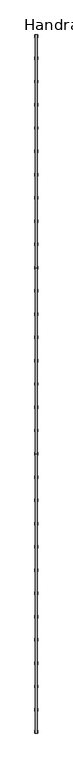
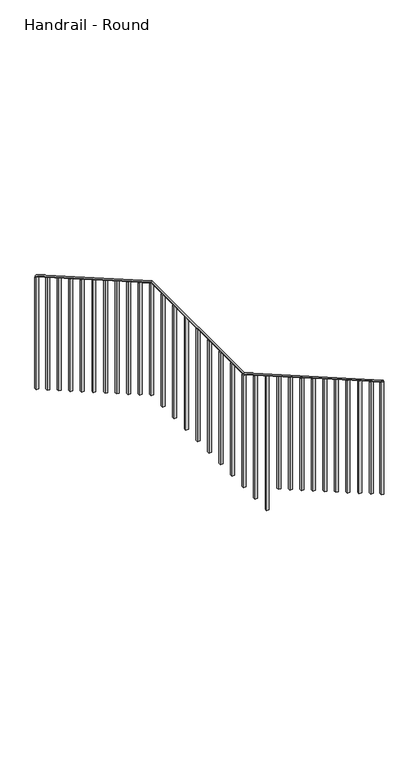
"""IFC4 building model written with IfcOpenShell, lengths in millimetres: railing geometry, Handrail - Round."""

import ifcopenshell
import ifcopenshell.guid

model = None  # the IFC model being written
_history = None  # IfcOwnerHistory: only IFC2X3 demands one
_inside = {}  # id of a spatial element -> (the spatial element, [elements in it])
_under = {}  # id of a project, library or spatial element -> (it, [spatial elements below it])
_declared = {}  # id of a project -> (the project, [libraries it declares])
_typed = {}  # id of a type object -> (the type object, [elements of that type])
_made_of = {}  # id of a material, layer set ... -> (it, [elements and type objects made of it])


def new_model(schema):
    """Start an empty IFC model of exactly this schema.

    Asked for "IFC4X3", IfcOpenShell would pick the latest addendum, in which some entities
    have other attributes; the version numbers below select the first issue.
    IFC2X3 requires an IfcOwnerHistory on every rooted entity: one is made here for all.
    """
    global model, _history
    if schema == "IFC4X3":
        model = ifcopenshell.file(schema_version=(4, 3, 0, 0))
    else:
        model = ifcopenshell.file(schema=schema)
    _inside.clear()
    _under.clear()
    _declared.clear()
    _typed.clear()
    _made_of.clear()
    _history = None
    if model.schema == "IFC2X3":
        org = make("IfcOrganization", Name="unknown")
        user = make(
            "IfcPersonAndOrganization",
            ThePerson=make("IfcPerson", FamilyName="unknown"),
            TheOrganization=org,
        )
        app = make(
            "IfcApplication",
            ApplicationDeveloper=org,
            Version="unknown",
            ApplicationFullName="unknown",
            ApplicationIdentifier="unknown",
        )
        _history = make(
            "IfcOwnerHistory",
            OwningUser=user,
            OwningApplication=app,
            ChangeAction="ADDED",
            CreationDate=0,
        )
    return model


def make(cls, **values):
    """One entity of the class cls with the attributes given. An attribute that is None is left unset."""
    return model.create_entity(
        cls, **{name: value for name, value in values.items() if value is not None}
    )


def rooted(cls, **values):
    """An entity with a GlobalId (a new one), such as an element, a storey or a relation."""
    return make(cls, GlobalId=ifcopenshell.guid.new(), OwnerHistory=_history, **values)


def si_unit(unit_type, name, prefix=None):
    """IfcSIUnit, for example si_unit("LENGTHUNIT", "METRE", prefix="MILLI")."""
    return make("IfcSIUnit", UnitType=unit_type, Prefix=prefix, Name=name)


def assignment(units):
    """IfcUnitAssignment: the units of a project."""
    return None if units is None else make("IfcUnitAssignment", Units=units)


def point(xyz):
    """IfcCartesianPoint."""
    return None if xyz is None else make("IfcCartesianPoint", Coordinates=xyz)


def direction(xyz):
    """IfcDirection."""
    return None if xyz is None else make("IfcDirection", DirectionRatios=xyz)


def frame(location, z_axis=None, x_axis=None):
    """IfcAxis2Placement3D, a coordinate frame: its origin and axes. An axis left out is left unset."""
    return make(
        "IfcAxis2Placement3D",
        Location=point(location),
        Axis=direction(z_axis),
        RefDirection=direction(x_axis),
    )


def origin():
    """The frame at (0, 0, 0) with its axes left unset."""
    return frame((0.0, 0.0, 0.0))


def place(relative_to, where):
    """IfcLocalPlacement: puts the frame where relative to a parent placement (None: the world)."""
    return make(
        "IfcLocalPlacement", PlacementRelTo=relative_to, RelativePlacement=where
    )


def context(
    kind, dimensions, precision=None, world=None, true_north=None, identifier=None
):
    """IfcGeometricRepresentationContext, for example the 3D "Model" context."""
    return make(
        "IfcGeometricRepresentationContext",
        ContextIdentifier=identifier,
        ContextType=kind,
        CoordinateSpaceDimension=dimensions,
        Precision=precision,
        WorldCoordinateSystem=world,
        TrueNorth=true_north,
    )


def project(units=None, contexts=None):
    """IfcProject with its units and contexts."""
    return rooted(
        "IfcProject",
        Name="project",
        RepresentationContexts=contexts,
        UnitsInContext=assignment(units),
    )


def spatial(cls, under=None, at=None, **own):
    """A site, building, storey or space (cls), placed at a placement, below another one or the project."""
    s = rooted(cls, ObjectPlacement=at, **own)
    if under is not None:
        _under.setdefault(under.id(), (under, []))[1].append(s)
    return s


def polyline(points):
    """IfcPolyline through the points."""
    return make("IfcPolyline", Points=[point(p) for p in points])


def ellipse_curve(where, semi_axis1, semi_axis2):
    """IfcEllipse in the frame where."""
    return make(
        "IfcEllipse", Position=where, SemiAxis1=semi_axis1, SemiAxis2=semi_axis2
    )


def outline(outer, holes=None, kind="AREA"):
    """IfcArbitraryClosedProfileDef: a profile drawn as a closed curve; with holes, ...WithVoids."""
    if holes is None:
        return make("IfcArbitraryClosedProfileDef", ProfileType=kind, OuterCurve=outer)
    return make(
        "IfcArbitraryProfileDefWithVoids",
        ProfileType=kind,
        OuterCurve=outer,
        InnerCurves=holes,
    )


def extrude(swept, where, along, depth):
    """IfcExtrudedAreaSolid: the profile swept, set in the frame where, extruded along a direction by depth."""
    return make(
        "IfcExtrudedAreaSolid",
        SweptArea=swept,
        Position=where,
        ExtrudedDirection=direction(along),
        Depth=depth,
    )


def shape(context_of_items, identifier, shape_type, items):
    """IfcShapeRepresentation: the items that make up one representation, for example the "Body"."""
    return make(
        "IfcShapeRepresentation",
        ContextOfItems=context_of_items,
        RepresentationIdentifier=identifier,
        RepresentationType=shape_type,
        Items=items,
    )


def source(mapping_origin, context_of_items, identifier, shape_type, items):
    """IfcRepresentationMap: a shape defined once, which mapped items show again and again."""
    return make(
        "IfcRepresentationMap",
        MappingOrigin=mapping_origin,
        MappedRepresentation=shape(context_of_items, identifier, shape_type, items),
    )


def transform(
    local_origin,
    x_axis=None,
    y_axis=None,
    z_axis=None,
    scale=None,
    scale2=None,
    scale3=None,
    uniform=True,
):
    """IfcCartesianTransformationOperator3D, or its non-uniform kind. x_axis, y_axis, z_axis: its Axis1, 2, 3."""
    if uniform:
        return make(
            "IfcCartesianTransformationOperator3D",
            Axis1=direction(x_axis),
            Axis2=direction(y_axis),
            LocalOrigin=point(local_origin),
            Scale=scale,
            Axis3=direction(z_axis),
        )
    return make(
        "IfcCartesianTransformationOperator3DnonUniform",
        Axis1=direction(x_axis),
        Axis2=direction(y_axis),
        LocalOrigin=point(local_origin),
        Scale=scale,
        Axis3=direction(z_axis),
        Scale2=scale2,
        Scale3=scale3,
    )


def mapped(mapping_source, mapping_target):
    """IfcMappedItem: shows the shape of a source again, moved by a transform."""
    return make(
        "IfcMappedItem", MappingSource=mapping_source, MappingTarget=mapping_target
    )


def made_of(thing, what):
    """Note that an element or type object is made of a material, layer set ...; save() writes the relation."""
    if what is not None:
        _made_of.setdefault(what.id(), (what, []))[1].append(thing)
    return thing


def element(
    cls,
    number,
    at=None,
    inside=None,
    cuts=None,
    type_object=None,
    material=None,
    context=None,
    identifier="Body",
    shape_type=None,
    held_by="IfcProductDefinitionShape",
    body=None,
    shapes=None,
    **own,
):
    """One element of the class cls, such as IfcWall. Its Tag is "e" and its number.

    at: its placement. inside: the storey or other place that contains it. cuts: it is an
    opening in that element (IfcRelVoidsElement). A single representation is given by context,
    identifier, shape_type and body (its items); several are given by shapes. held_by: the class
    of the entity that holds the representations. save() writes the other relations.
    """
    e = rooted(cls, Tag="e%d" % number, ObjectPlacement=at, **own)
    if body is not None:
        shapes = [shape(context, identifier, shape_type, body)]
    if shapes is not None:
        e.Representation = make(held_by, Representations=shapes)
    if inside is not None:
        _inside.setdefault(inside.id(), (inside, []))[1].append(e)
    if cuts is not None:
        rooted(
            "IfcRelVoidsElement", RelatingBuildingElement=cuts, RelatedOpeningElement=e
        )
    if type_object is not None:
        _typed.setdefault(type_object.id(), (type_object, []))[1].append(e)
    return made_of(e, material)


def aggregate(whole, parts):
    """IfcRelAggregates: a whole, such as a stair, and the parts it consists of."""
    return rooted("IfcRelAggregates", RelatingObject=whole, RelatedObjects=parts)


def save(model, path):
    """Write the relations noted so far, then the file.

    IfcRelAggregates (storeys below a building ...), IfcRelContainedInSpatialStructure (elements
    in a storey), IfcRelDefinesByType, IfcRelAssociatesMaterial and IfcRelDeclares: one each for
    every whole, place, type object, material and project.
    """
    for whole, parts in _under.values():
        aggregate(whole, parts)
    for where, things in _inside.values():
        rooted(
            "IfcRelContainedInSpatialStructure",
            RelatedElements=things,
            RelatingStructure=where,
        )
    for kind, things in _typed.values():
        rooted("IfcRelDefinesByType", RelatedObjects=things, RelatingType=kind)
    for what, things in _made_of.values():
        rooted("IfcRelAssociatesMaterial", RelatedObjects=things, RelatingMaterial=what)
    for by, libraries in _declared.values():
        rooted("IfcRelDeclares", RelatingContext=by, RelatedDefinitions=libraries)
    model.write(path)


def plane_surface(at):
    """IfcPlane: the flat surface through the origin of the frame at, square to its z axis."""
    return make("IfcPlane", Position=at)


def cylinder_surface(at, radius):
    """IfcCylindricalSurface: all points at the distance radius from the z axis of the frame at."""
    return make("IfcCylindricalSurface", Position=at, Radius=radius)


def advanced_brep(points, edges, surfaces, faces):
    """IfcAdvancedBrep: a solid bounded by faces that lie on surfaces and meet in shared edges.

    An edge is (start, end): straight between two places in points (the first is 0);
    or (start, end, curve); or (start, end, curve, False) where it runs against its curve.
    A face is (place in surfaces, loops), or (place, loops, False) where it looks against
    its surface's normal. A loop lists edges by number (the first is 1), with a minus sign
    where the edge is run from its end to its start. The first loop is the outer one.
    """
    corners = [point(p) for p in points]
    vertices = [make("IfcVertexPoint", VertexGeometry=c) for c in corners]
    made = []
    for start, end, *more in edges:
        made.append(
            make(
                "IfcEdgeCurve",
                EdgeStart=vertices[start],
                EdgeEnd=vertices[end],
                EdgeGeometry=more[0] if more else make("IfcPolyline", Points=[corners[start], corners[end]]),
                SameSense=more[1] if len(more) > 1 else True,
            )
        )
    hull = []
    for where, loops, *sense in faces:
        bounds = []
        for j, loop in enumerate(loops):
            ring = [make("IfcOrientedEdge", EdgeElement=made[abs(k) - 1], Orientation=k > 0) for k in loop]
            bounds.append(
                make(
                    "IfcFaceOuterBound" if j == 0 else "IfcFaceBound",
                    Bound=make("IfcEdgeLoop", EdgeList=ring),
                    Orientation=True,
                )
            )
        hull.append(make("IfcAdvancedFace", Bounds=bounds, FaceSurface=surfaces[where], SameSense=sense[0] if sense else True))
    return make("IfcAdvancedBrep", Outer=make("IfcClosedShell", CfsFaces=hull))


def handrail_round_a1da8104(model_context):
    return source(origin(), model_context, "Body", "SolidModel", [
        advanced_brep(
        [(-88495.1875, 4699.0, 12273.5609368), (-88482.4875, 4699.0, 12273.5609368), (-88495.1875, 127.0, 14200.5991721), (-88482.4875, 127.0, 14200.5991721), (-88495.1875, 3173.3051523, 13150.4615294), (-88482.4875, 3173.3051523, 13150.4615294), (-88495.1875, 1954.1051523, 13150.4615294), (-88482.4875, 1954.1051523, 13150.4615294)],
        [
            (0, 1, ellipse_curve(frame((-88488.8375, 4699.0, 12273.5609368), z_axis=(0.0, 1.0, 0.0), x_axis=(0.0, 0.0, -1.0)), 7.324122, 6.35)),
            (1, 0, ellipse_curve(frame((-88488.8375, 4699.0, 12273.5609368), z_axis=(0.0, 1.0, 0.0), x_axis=(0.0, 0.0, -1.0)), 7.324122, 6.35)),
            (2, 3, ellipse_curve(frame((-88488.8375, 127.0, 14200.5991721), z_axis=(0.0, -1.0, 0.0), x_axis=(0.0, 0.0, -1.0)), 7.324122, 6.35)),
            (3, 2, ellipse_curve(frame((-88488.8375, 127.0, 14200.5991721), z_axis=(0.0, -1.0, 0.0), x_axis=(0.0, 0.0, -1.0)), 7.324122, 6.35)),
            (0, 4),
            (4, 5, ellipse_curve(frame((-88488.8375, 3173.3051523, 13150.4615294), z_axis=(0.0, 0.9661775497539637, -0.2578777662991265), x_axis=(0.0, -0.2578777662991264, -0.9661775497539637)), 6.572291, 6.35)),
            (5, 1),
            (5, 4, ellipse_curve(frame((-88488.8375, 3173.3051523, 13150.4615294), z_axis=(0.0, 0.9661775497539637, -0.2578777662991265), x_axis=(0.0, -0.2578777662991264, -0.9661775497539637)), 6.572291, 6.35)),
            (4, 6),
            (6, 7, ellipse_curve(frame((-88488.8375, 1954.1051523, 13150.4615294), z_axis=(0.0, 0.9661775497539637, -0.2578777662991265), x_axis=(0.0, 0.25787776629912645, 0.9661775497539637)), 6.572291, 6.35)),
            (7, 5),
            (7, 6, ellipse_curve(frame((-88488.8375, 1954.1051523, 13150.4615294), z_axis=(0.0, 0.9661775497539637, -0.2578777662991265), x_axis=(0.0, 0.25787776629912645, 0.9661775497539637)), 6.572291, 6.35)),
            (6, 2),
            (3, 7),
        ],
        [
            plane_surface(frame((-88488.8375, 4699.0, 12280.8850588), z_axis=(0.0, 1.0, 0.0), x_axis=(0.0, 0.0, -1.0))),
            plane_surface(frame((-88488.8375, 127.0, 14207.9232941), z_axis=(0.0, -1.0, 0.0), x_axis=(0.0, 0.0, -1.0))),
            cylinder_surface(frame((-88488.8375, 4695.8357225, 12275.3796208), z_axis=(0.0, 0.8669981152971462, -0.49831141675783075), x_axis=(1.0, 0.0, 0.0)), 6.35),
            cylinder_surface(frame((-88488.8375, 3175.0, 13150.4615294), z_axis=(0.0, 1.0, 0.0), x_axis=(1.0, 0.0, 0.0)), 6.35),
            cylinder_surface(frame((-88488.8375, 1952.6357225, 13151.3060914), z_axis=(0.0, 0.8669981152971462, -0.4983114167578307), x_axis=(1.0, 0.0, 0.0)), 6.35),
        ],
        [
            (0, [[1, 2]]),
            (1, [[3, 4]]),
            (2, [[-1, 5, 6, 7]]),
            (2, [[-2, -7, 8, -5]]),
            (3, [[-6, 9, 10, 11]]),
            (3, [[-8, -11, 12, -9]]),
            (4, [[-10, 13, -4, 14]]),
            (4, [[-12, -14, -3, -13]]),
        ],
    ),
        extrude(outline(polyline([(288.925, 14100.2078625), (288.925, 13205.9306471), (269.875, 13205.9306471), (269.875, 14111.1569434), (288.925, 14100.2078625)])), frame((-88498.3625, 0.0, 0.0), z_axis=(1.0, 0.0, 0.0), x_axis=(0.0, 1.0, 0.0)), (0.0, 0.0, 1.0), 19.05),
        extrude(outline(polyline([(441.325, 14012.6152155), (441.325, 13118.338), (422.275, 13118.338), (422.275, 14023.5642964), (441.325, 14012.6152155)])), frame((-88498.3625, 0.0, 0.0), z_axis=(1.0, 0.0, 0.0), x_axis=(0.0, 1.0, 0.0)), (0.0, 0.0, 1.0), 19.05),
        extrude(outline(polyline([(593.725, 13925.0225684), (593.725, 13030.7453529), (574.675, 13030.7453529), (574.675, 13935.9716493), (593.725, 13925.0225684)])), frame((-88498.3625, 0.0, 0.0), z_axis=(1.0, 0.0, 0.0), x_axis=(0.0, 1.0, 0.0)), (0.0, 0.0, 1.0), 19.05),
        extrude(outline(polyline([(746.125, 13837.4299214), (746.125, 12943.1527059), (727.075, 12943.1527059), (727.075, 13848.3790023), (746.125, 13837.4299214)])), frame((-88498.3625, 0.0, 0.0), z_axis=(1.0, 0.0, 0.0), x_axis=(0.0, 1.0, 0.0)), (0.0, 0.0, 1.0), 19.05),
        extrude(outline(polyline([(898.525, 13749.8372743), (898.525, 12855.5600588), (879.475, 12855.5600588), (879.475, 13760.7863552), (898.525, 13749.8372743)])), frame((-88498.3625, 0.0, 0.0), z_axis=(1.0, 0.0, 0.0), x_axis=(0.0, 1.0, 0.0)), (0.0, 0.0, 1.0), 19.05),
        extrude(outline(polyline([(1050.925, 13662.2446273), (1050.925, 12767.9674118), (1031.875, 12767.9674118), (1031.875, 13673.1937081), (1050.925, 13662.2446273)])), frame((-88498.3625, 0.0, 0.0), z_axis=(1.0, 0.0, 0.0), x_axis=(0.0, 1.0, 0.0)), (0.0, 0.0, 1.0), 19.05),
        extrude(outline(polyline([(1203.325, 13574.6519802), (1203.325, 12680.3747647), (1184.275, 12680.3747647), (1184.275, 13585.6010611), (1203.325, 13574.6519802)])), frame((-88498.3625, 0.0, 0.0), z_axis=(1.0, 0.0, 0.0), x_axis=(0.0, 1.0, 0.0)), (0.0, 0.0, 1.0), 19.05),
        extrude(outline(polyline([(1355.725, 13487.0593331), (1355.725, 12592.7821176), (1336.675, 12592.7821176), (1336.675, 13498.008414), (1355.725, 13487.0593331)])), frame((-88498.3625, 0.0, 0.0), z_axis=(1.0, 0.0, 0.0), x_axis=(0.0, 1.0, 0.0)), (0.0, 0.0, 1.0), 19.05),
        extrude(outline(polyline([(1508.125, 13399.4666861), (1508.125, 12505.1894706), (1489.075, 12505.1894706), (1489.075, 13410.415767), (1508.125, 13399.4666861)])), frame((-88498.3625, 0.0, 0.0), z_axis=(1.0, 0.0, 0.0), x_axis=(0.0, 1.0, 0.0)), (0.0, 0.0, 1.0), 19.05),
        extrude(outline(polyline([(1660.525, 13311.874039), (1660.525, 12242.4115294), (1641.475, 12242.4115294), (1641.475, 13322.8231199), (1660.525, 13311.874039)])), frame((-88498.3625, 0.0, 0.0), z_axis=(1.0, 0.0, 0.0), x_axis=(0.0, 1.0, 0.0)), (0.0, 0.0, 1.0), 19.05),
        extrude(outline(polyline([(1812.925, 13224.281392), (1812.925, 12242.4115294), (1793.875, 12242.4115294), (1793.875, 13235.2304728), (1812.925, 13224.281392)])), frame((-88498.3625, 0.0, 0.0), z_axis=(1.0, 0.0, 0.0), x_axis=(0.0, 1.0, 0.0)), (0.0, 0.0, 1.0), 19.05),
        extrude(outline(polyline([(-88479.3125, 2117.725), (-88479.3125, 2098.675), (-88498.3625, 2098.675), (-88498.3625, 2117.725), (-88479.3125, 2117.725)])), frame((0.0, 0.0, 12242.4115294), z_axis=(0.0, 0.0, 1.0), x_axis=(1.0, 0.0, 0.0)), (0.0, 0.0, 1.0), 901.7),
        extrude(outline(polyline([(-88479.3125, 2270.125), (-88479.3125, 2251.075), (-88498.3625, 2251.075), (-88498.3625, 2270.125), (-88479.3125, 2270.125)])), frame((0.0, 0.0, 12242.4115294), z_axis=(0.0, 0.0, 1.0), x_axis=(1.0, 0.0, 0.0)), (0.0, 0.0, 1.0), 901.7),
        extrude(outline(polyline([(-88479.3125, 2422.525), (-88479.3125, 2403.475), (-88498.3625, 2403.475), (-88498.3625, 2422.525), (-88479.3125, 2422.525)])), frame((0.0, 0.0, 12242.4115294), z_axis=(0.0, 0.0, 1.0), x_axis=(1.0, 0.0, 0.0)), (0.0, 0.0, 1.0), 901.7),
        extrude(outline(polyline([(-88479.3125, 2574.925), (-88479.3125, 2555.875), (-88498.3625, 2555.875), (-88498.3625, 2574.925), (-88479.3125, 2574.925)])), frame((0.0, 0.0, 12242.4115294), z_axis=(0.0, 0.0, 1.0), x_axis=(1.0, 0.0, 0.0)), (0.0, 0.0, 1.0), 901.7),
        extrude(outline(polyline([(-88479.3125, 2727.325), (-88479.3125, 2708.275), (-88498.3625, 2708.275), (-88498.3625, 2727.325), (-88479.3125, 2727.325)])), frame((0.0, 0.0, 12242.4115294), z_axis=(0.0, 0.0, 1.0), x_axis=(1.0, 0.0, 0.0)), (0.0, 0.0, 1.0), 901.7),
        extrude(outline(polyline([(-88479.3125, 2879.725), (-88479.3125, 2860.675), (-88498.3625, 2860.675), (-88498.3625, 2879.725), (-88479.3125, 2879.725)])), frame((0.0, 0.0, 12242.4115294), z_axis=(0.0, 0.0, 1.0), x_axis=(1.0, 0.0, 0.0)), (0.0, 0.0, 1.0), 901.7),
        extrude(outline(polyline([(-88479.3125, 3032.125), (-88479.3125, 3013.075), (-88498.3625, 3013.075), (-88498.3625, 3032.125), (-88479.3125, 3032.125)])), frame((0.0, 0.0, 12242.4115294), z_axis=(0.0, 0.0, 1.0), x_axis=(1.0, 0.0, 0.0)), (0.0, 0.0, 1.0), 901.7),
        extrude(outline(polyline([(3336.925, 13049.0960978), (3336.925, 12154.8188824), (3317.875, 12154.8188824), (3317.875, 13060.0451787), (3336.925, 13049.0960978)])), frame((-88498.3625, 0.0, 0.0), z_axis=(1.0, 0.0, 0.0), x_axis=(0.0, 1.0, 0.0)), (0.0, 0.0, 1.0), 19.05),
        extrude(outline(polyline([(3489.325, 12961.5034508), (3489.325, 12067.2262353), (3470.275, 12067.2262353), (3470.275, 12972.4525317), (3489.325, 12961.5034508)])), frame((-88498.3625, 0.0, 0.0), z_axis=(1.0, 0.0, 0.0), x_axis=(0.0, 1.0, 0.0)), (0.0, 0.0, 1.0), 19.05),
        extrude(outline(polyline([(3641.725, 12873.9108037), (3641.725, 11979.6335882), (3622.675, 11979.6335882), (3622.675, 12884.8598846), (3641.725, 12873.9108037)])), frame((-88498.3625, 0.0, 0.0), z_axis=(1.0, 0.0, 0.0), x_axis=(0.0, 1.0, 0.0)), (0.0, 0.0, 1.0), 19.05),
        extrude(outline(polyline([(3794.125, 12786.3181567), (3794.125, 11892.0409412), (3775.075, 11892.0409412), (3775.075, 12797.2672375), (3794.125, 12786.3181567)])), frame((-88498.3625, 0.0, 0.0), z_axis=(1.0, 0.0, 0.0), x_axis=(0.0, 1.0, 0.0)), (0.0, 0.0, 1.0), 19.05),
        extrude(outline(polyline([(3946.525, 12698.7255096), (3946.525, 11804.4482941), (3927.475, 11804.4482941), (3927.475, 12709.6745905), (3946.525, 12698.7255096)])), frame((-88498.3625, 0.0, 0.0), z_axis=(1.0, 0.0, 0.0), x_axis=(0.0, 1.0, 0.0)), (0.0, 0.0, 1.0), 19.05),
        extrude(outline(polyline([(4098.925, 12611.1328625), (4098.925, 11716.8556471), (4079.875, 11716.8556471), (4079.875, 12622.0819434), (4098.925, 12611.1328625)])), frame((-88498.3625, 0.0, 0.0), z_axis=(1.0, 0.0, 0.0), x_axis=(0.0, 1.0, 0.0)), (0.0, 0.0, 1.0), 19.05),
        extrude(outline(polyline([(4251.325, 12523.5402155), (4251.325, 11629.263), (4232.275, 11629.263), (4232.275, 12534.4892964), (4251.325, 12523.5402155)])), frame((-88498.3625, 0.0, 0.0), z_axis=(1.0, 0.0, 0.0), x_axis=(0.0, 1.0, 0.0)), (0.0, 0.0, 1.0), 19.05),
        extrude(outline(polyline([(4403.725, 12435.9475684), (4403.725, 11541.6703529), (4384.675, 11541.6703529), (4384.675, 12446.8966493), (4403.725, 12435.9475684)])), frame((-88498.3625, 0.0, 0.0), z_axis=(1.0, 0.0, 0.0), x_axis=(0.0, 1.0, 0.0)), (0.0, 0.0, 1.0), 19.05),
        extrude(outline(polyline([(4556.125, 12348.3549214), (4556.125, 11454.0777059), (4537.075, 11454.0777059), (4537.075, 12359.3040023), (4556.125, 12348.3549214)])), frame((-88498.3625, 0.0, 0.0), z_axis=(1.0, 0.0, 0.0), x_axis=(0.0, 1.0, 0.0)), (0.0, 0.0, 1.0), 19.05),
        extrude(outline(polyline([(-88479.3125, 1965.325), (-88479.3125, 1946.275), (-88498.3625, 1946.275), (-88498.3625, 1965.325), (-88479.3125, 1965.325)])), frame((0.0, 0.0, 12242.4115294), z_axis=(0.0, 0.0, 1.0), x_axis=(1.0, 0.0, 0.0)), (0.0, 0.0, 1.0), 901.7),
        extrude(outline(polyline([(3184.525, 13136.6887449), (3184.525, 12242.4115294), (3165.475, 12242.4115294), (3165.475, 13147.6378258), (3184.525, 13136.6887449)])), frame((-88498.3625, 0.0, 0.0), z_axis=(1.0, 0.0, 0.0), x_axis=(0.0, 1.0, 0.0)), (0.0, 0.0, 1.0), 19.05),
        extrude(outline(polyline([(146.05, 14182.3259692), (146.05, 13288.0487537), (127.0, 13288.0487537), (127.0, 14193.27505), (146.05, 14182.3259692)])), frame((-88498.3625, 0.0, 0.0), z_axis=(1.0, 0.0, 0.0), x_axis=(0.0, 1.0, 0.0)), (0.0, 0.0, 1.0), 19.05),
        extrude(outline(polyline([(4699.0, 12266.2368148), (4699.0, 11371.9595993), (4679.95, 11371.9595993), (4679.95, 12277.1858956), (4699.0, 12266.2368148)])), frame((-88498.3625, 0.0, 0.0), z_axis=(1.0, 0.0, 0.0), x_axis=(0.0, 1.0, 0.0)), (0.0, 0.0, 1.0), 19.05),
    ])


if __name__ == "__main__":
    model = new_model("IFC4")
    model_context = context("Model", 3, world=origin())
    ifc_project = project(units=[si_unit("LENGTHUNIT", "METRE", prefix="MILLI")], contexts=[model_context])
    site = spatial("IfcSite", under=ifc_project)
    building = spatial("IfcBuilding", under=site)
    placement = place(None, origin())
    handrail_round_shape = handrail_round_a1da8104(model_context)
    element("IfcRailing", 1, ObjectType="Handrail - Round", at=placement, inside=building, context=model_context, shape_type="MappedRepresentation", body=[
        mapped(handrail_round_shape, transform((0.0, 0.0, 0.0), x_axis=(1.0, 0.0, 0.0), y_axis=(0.0, 1.0, 0.0), z_axis=(0.0, 0.0, 1.0))),
    ])
    save(model, "model.ifc")
